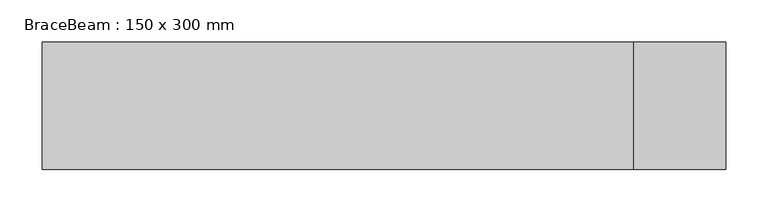
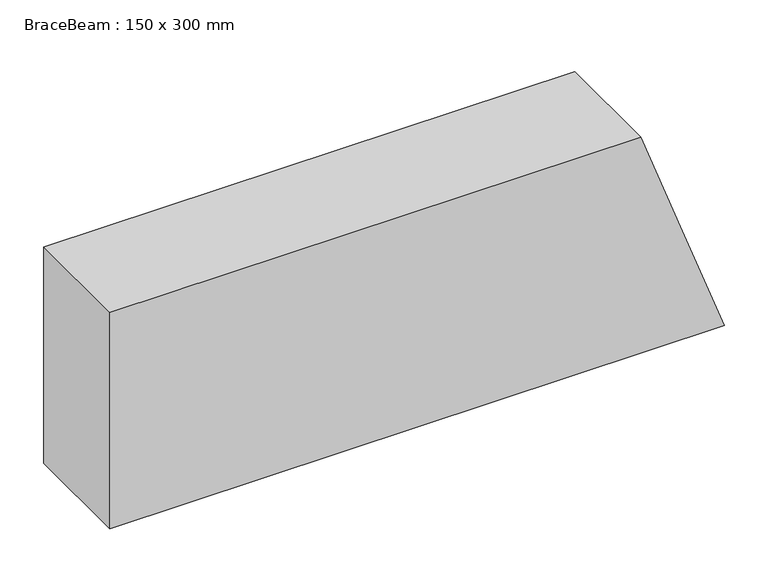
"""IFC4 building model written with IfcOpenShell, lengths in millimetres: beam geometry, BraceBeam : 150 x 300 mm."""

from ifc_helpers import new_model, si_unit, origin, place, context, project, spatial, faceted_brep, source, transform, mapped, element, save


def bracebeam_150_x_300_mm_91503ad9(model_context):
    return source(origin(), model_context, "Body", "Brep", [
        faceted_brep([(-380.4256539, -75.0, -150.0), (-380.4256539, 75.0, -150.0), (425.3945231, 75.0, -150.0), (425.3945231, -75.0, -150.0), (-380.4256539, 75.0, 150.0), (316.2034529, 75.0, 150.0), (370.798988, 75.0, 0.0), (-380.4256539, -75.0, 150.0), (316.2034529, -75.0, 150.0), (370.798988, -75.0, 0.0)], [[[0, 1, 2, 3]], [[1, 4, 5, 6, 2]], [[4, 7, 8, 5]], [[7, 0, 3, 9, 8]], [[7, 4, 1, 0]], [[5, 8, 9, 3, 2, 6]]]),
    ])


if __name__ == "__main__":
    model = new_model("IFC4")
    model_context = context("Model", 3, world=origin())
    ifc_project = project(units=[si_unit("LENGTHUNIT", "METRE", prefix="MILLI")], contexts=[model_context])
    site = spatial("IfcSite", under=ifc_project)
    building = spatial("IfcBuilding", under=site)
    placement = place(None, origin())
    bracebeam_150_x_300_mm_shape = bracebeam_150_x_300_mm_91503ad9(model_context)
    element("IfcBeam", 1, ObjectType="BraceBeam : 150 x 300 mm", at=placement, inside=building, context=model_context, shape_type="MappedRepresentation", body=[
        mapped(bracebeam_150_x_300_mm_shape, transform((0.0, 0.0, 0.0), x_axis=(1.0, 0.0, 0.0), y_axis=(0.0, 1.0, 0.0), z_axis=(0.0, 0.0, 1.0))),
    ])
    save(model, "model.ifc")

# Revit data of these elements
# Type "BraceBeam : 150 x 300 mm"
#   ExpertTruss = "Height\th\r\nWidth\tb"
#   Name [instance default] = ""
#   m [instance default] = 0 mm
#   ip_c_cut_control [instance default] = 1300 mm
#   ip_c_cut [instance default] = 1300 mm
#   h_fix [instance default] = 900 mm
#   d/2 [instance default] = 1750 mm
#   c_cut_incl [instance default] = -1000 mm
#   c_cut [instance default] = 0 mm
#   beta0_2 [instance default] = 90.00°
#   beta0_1 [instance default] = 90.00°
#   alfaMax [instance default] = 0.00°
#   alfa0_2 [instance default] = 90.00°
#   ZOffsetStr_0 [instance default] = 150 mm
#   ZOffsetStr [instance default] = 0 mm
#   ZOffsetEnd_0 [instance default] = 150 mm
#   ZOffsetEnd [instance default] = 0 mm
#   Beta2 [instance default] = 0.00°
#   Beta1 [instance default] = 0.00°
#   Alfa_str [instance default] = 0.00°
#   Alfa_cut_control [instance default] = 90.00°
#   Alfa_cut [instance default] = 90.00°
#   AlfaMAX [instance default] = 0.00°
#   Alfa2_0 [instance default] = 0.00°
#   Alfa2 [instance default] = 0.00°
#   Alfa1_0 [instance default] = 0.00°
#   Alfa1 [instance default] = 0.00°
#   A_max_Str [instance default] = 0.00°
#   h_void [instance default] = 3000 mm
#   beam_L_0 [instance default] = 100 mm
#   beam_L [instance default] = 0 mm
#   b_void [instance default] = 160 mm
#   alfa0_1 [instance default] = 90.00°
#   b = 150 mm
#   YOffsetStr [instance default] = 0 mm
#   YOffsetEnd [instance default] = 0 mm
#   XOffsetStr_0 [instance default] = 3500 mm
#   XOffsetStr [instance default] = 0 mm
#   XOffsetEnd_0 [instance default] = 3500 mm
#   XOffsetEnd [instance default] = 0 mm
#   L_void_0 [instance default] = 100 mm
#   L_void [instance default] = 0 mm
#   E2 [instance default] = 0.00°
#   E1 [instance default] = 0.00°
#   Length [instance default] = 3500 mm
#   h = 300 mm
#   Alfa [instance default] = 0.00°
#   A_max_End [instance default] = 0.00°
#   A_max [instance default] = 0.00°
#   A4 [instance default] = 0.00°
#   A3 [instance default] = 0.00°
#   A2 [instance default] = 0.00°
#   A1 [instance default] = 0.00°
#   BetaAngles [instance default] = no
#   Material [instance default] = Wood Standard
# Element 1 (IfcBeam, "BraceBeam : 150 x 300 mm")
#   d/2 = 535.067 mm
#   beta0_2 = 70.00°
#   alfaMax = -20.00°
#   alfa0_2 = 70.00°
#   AlfaMAX = -20.00°
#   Alfa2_0 = -20.00°
#   Alfa2 = -20.00°
#   h_void = 4091.911 mm
#   beam_L_0 = 873.529 mm
#   beam_L = 873.529 mm
#   XOffsetStr_0 = 920.134 mm
#   XOffsetStr = 150 mm
#   XOffsetEnd_0 = 910.507 mm
#   XOffsetEnd = 159.627 mm
#   L_void_0 = 2064.996 mm
#   L_void = 2064.996 mm
#   Materials on its faces: "Wood Standard"
# Materials
#   "Wood Standard": class "Drewno", colour RGB 196 146 67, transparency 0, Cost = 0
